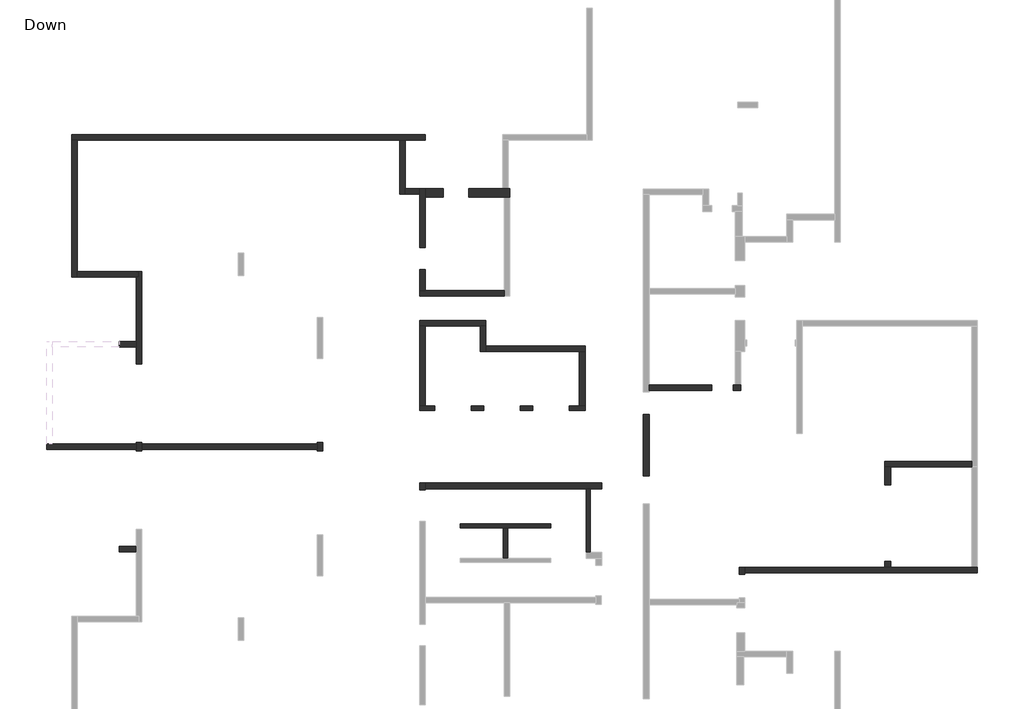
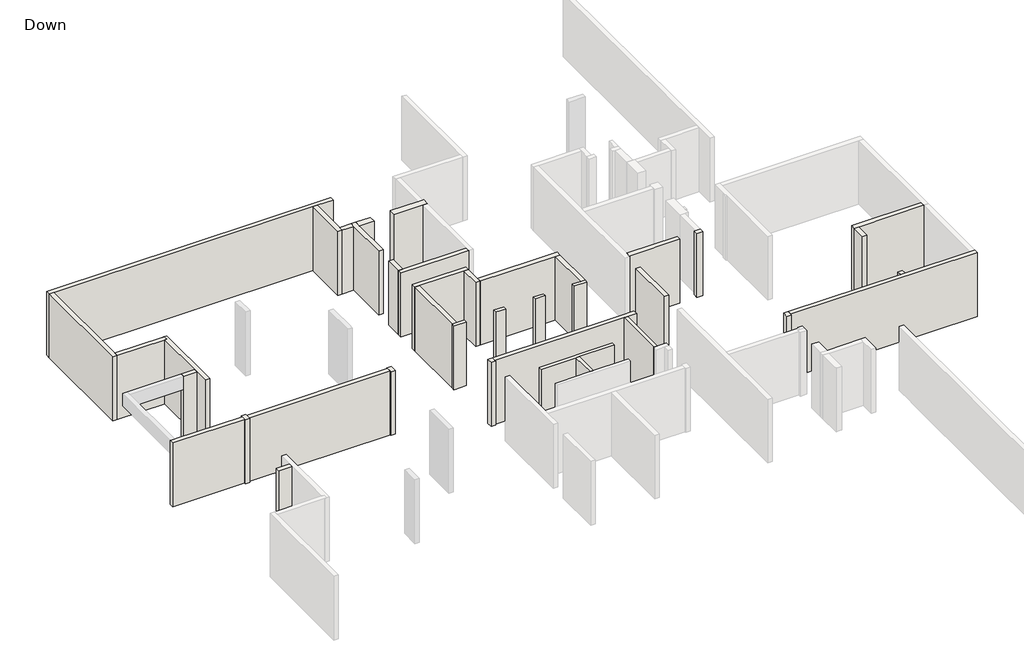
# One storey, part 2 of 3: 39 walls.
"""IFC4 building model written with IfcOpenShell, lengths in millimetres."""

from ifc_helpers import new_model, si_unit, origin, origin_with_axes, place, context, project, spatial, polyline, outline, extrude, faceted_brep, element, save

model = new_model("IFC4")

# Units and contexts
model_context = context("Model", 3, world=origin())
ifc_project = project(units=[si_unit("LENGTHUNIT", "METRE", prefix="MILLI")], contexts=[model_context])

# Site, building, storey
site = spatial("IfcSite", under=ifc_project)
building = spatial("IfcBuilding", under=site)
storey = spatial("IfcBuildingStorey", under=building, Name="Down", Elevation=0.0)

# Walls
placement = place(None, origin())
element("IfcWall", 1, ObjectType="15", at=placement, inside=storey, context=model_context, shape_type="Brep", body=[
    faceted_brep([(3274.3005639, 5124.0243454, 0.0), (3074.3005639, 5124.0243454, 0.0), (2715.3310352, 5124.0243454, 0.0), (2715.3310352, 5124.0243454, 2800.0), (2715.3310352, 5124.0243454, 3000.0), (3074.3005639, 5124.0243454, 3000.0), (3274.3005639, 5124.0243454, 3000.0), (3274.3005639, 4974.0243454, 0.0), (3274.3005639, 4974.0243454, 2800.0), (3274.3005639, 4974.0243454, 3000.0), (2715.3310352, 4974.0243454, 3000.0), (2715.3310352, 4974.0243454, 2800.0), (2715.3310352, 4974.0243454, 0.0)], [[[0, 1, 2, 3, 4, 5, 6]], [[7, 8, 9, 10, 11, 12]], [[2, 1, 0, 7, 12]], [[4, 3, 2, 12, 11, 10]], [[6, 5, 4, 10, 9]], [[0, 6, 9, 8, 7]]]),
])
element("IfcWall", 2, ObjectType="15", at=placement, inside=storey, context=model_context, shape_type="Brep", body=[
    faceted_brep([(1414.2577839, 5124.0243454, 0.0), (966.2691919, 5124.0243454, 0.0), (966.2691919, 5124.0243454, 2800.0), (966.2691919, 5124.0243454, 3000.0), (1414.2577839, 5124.0243454, 3000.0), (1414.2577839, 5124.0243454, 2800.0), (1414.2577839, 4974.0243454, 0.0), (1414.2577839, 4974.0243454, 2800.0), (1414.2577839, 4974.0243454, 3000.0), (966.2691919, 4974.0243454, 3000.0), (966.2691919, 4974.0243454, 2800.0), (966.2691919, 4974.0243454, 0.0)], [[[0, 1, 2, 3, 4, 5]], [[6, 7, 8, 9, 10, 11]], [[1, 0, 6, 11]], [[3, 2, 1, 11, 10, 9]], [[4, 3, 9, 8]], [[0, 5, 4, 8, 7, 6]]]),
])
element("IfcWall", 3, ObjectType="15", at=placement, inside=storey, context=model_context, shape_type="Brep", body=[
    faceted_brep([(-334.8040593, 5124.0243454, 0.0), (-785.1755694, 5124.0243454, 0.0), (-785.1755694, 5124.0243454, 2800.0), (-785.1755694, 5124.0243454, 3000.0), (-334.8040593, 5124.0243454, 3000.0), (-334.8040593, 5124.0243454, 2800.0), (-334.8040593, 4974.0243454, 0.0), (-334.8040593, 4974.0243454, 2800.0), (-334.8040593, 4974.0243454, 3000.0), (-785.1755694, 4974.0243454, 3000.0), (-785.1755694, 4974.0243454, 2800.0), (-785.1755694, 4974.0243454, 0.0)], [[[0, 1, 2, 3, 4, 5]], [[6, 7, 8, 9, 10, 11]], [[1, 0, 6, 11]], [[3, 2, 1, 11, 10, 9]], [[4, 3, 9, 8]], [[0, 5, 4, 8, 7, 6]]]),
])
element("IfcWall", 4, ObjectType="15", at=placement, inside=storey, context=model_context, shape_type="Brep", body=[
    faceted_brep([(-2083.8659026, 5124.0243454, 0.0), (-2434.3199705, 5124.0243454, 0.0), (-2634.3199705, 5124.0243454, 0.0), (-2634.3199705, 5124.0243454, 3000.0), (-2434.3199705, 5124.0243454, 3000.0), (-2083.8659026, 5124.0243454, 3000.0), (-2083.8659026, 5124.0243454, 2800.0), (-2083.8659026, 4974.0243454, 0.0), (-2083.8659026, 4974.0243454, 2800.0), (-2083.8659026, 4974.0243454, 3000.0), (-2634.3199705, 4974.0243454, 3000.0), (-2634.3199705, 4974.0243454, 2800.0), (-2634.3199705, 4974.0243454, 0.0)], [[[0, 1, 2, 3, 4, 5, 6]], [[7, 8, 9, 10, 11, 12]], [[2, 1, 0, 7, 12]], [[5, 4, 3, 10, 9]], [[0, 6, 5, 9, 8, 7]], [[3, 2, 12, 11, 10]]]),
])
element("IfcWall", 5, ObjectType="15", at=placement, inside=storey, context=model_context, shape_type="Brep", body=[
    faceted_brep([(3311.0605459, 2174.0956453, 0.0), (3311.0605459, -105.9043547, 0.0), (3311.0605459, -105.9043547, 3000.0), (3311.0605459, 2174.0956453, 3000.0), (3461.0605459, 2174.0956453, 0.0), (3461.0605459, 2174.0956453, 3000.0), (3461.0605459, -105.9043547, 3000.0), (3461.0605459, -105.9043547, 2800.0), (3461.0605459, -105.9043547, 0.0)], [[[0, 1, 2, 3]], [[4, 5, 6, 7, 8]], [[1, 0, 4, 8]], [[3, 2, 6, 5]], [[0, 3, 5, 4]], [[2, 1, 8, 7, 6]]]),
])
element("IfcWall", 6, ObjectType="15", at=placement, inside=storey, context=model_context, shape_type="Brep", body=[
    faceted_brep([(-1185.5058006, 773.063673, 0.0), (361.0080091, 773.063673, 0.0), (511.0080091, 773.063673, 0.0), (2055.2627374, 773.063673, 0.0), (2055.2627374, 773.063673, 2800.0), (2055.2627374, 773.063673, 3000.0), (1795.2627374, 773.063673, 3000.0), (511.0080091, 773.063673, 3000.0), (361.0080091, 773.063673, 3000.0), (-985.5058006, 773.063673, 3000.0), (-1185.5058006, 773.063673, 3000.0), (-1185.5058006, 773.063673, 2800.0), (-1185.5058006, 923.063673, 0.0), (-1185.5058006, 923.063673, 2800.0), (-1185.5058006, 923.063673, 3000.0), (2055.2627374, 923.063673, 3000.0), (2055.2627374, 923.063673, 2800.0), (2055.2627374, 923.063673, 0.0)], [[[0, 1, 2, 3, 4, 5, 6, 7, 8, 9, 10, 11]], [[12, 13, 14, 15, 16, 17]], [[3, 2, 1, 0, 12, 17]], [[5, 4, 3, 17, 16, 15]], [[10, 9, 8, 7, 6, 5, 15, 14]], [[0, 11, 10, 14, 13, 12]]]),
])
element("IfcWall", 7, ObjectType="15", at=placement, inside=storey, context=model_context, shape_type="SweptSolid", body=[
    extrude(outline(polyline([(511.0080091, 773.063673), (511.0080091, -306.6458737), (361.0080091, -306.6458737), (361.0080091, 773.063673), (511.0080091, 773.063673)])), origin_with_axes(), (0.0, 0.0, 1.0), 3000.0),
])
element("IfcWall", 8, ObjectType="20", at=placement, inside=storey, context=model_context, shape_type="Brep", body=[
    faceted_brep([(5555.6042265, 5674.60225, 0.0), (7795.7123021, 5674.60225, 0.0), (7795.7123021, 5674.60225, 2800.0), (7795.7123021, 5674.60225, 3000.0), (5555.6042265, 5674.60225, 3000.0), (5555.6042265, 5674.60225, 2800.0), (5555.6042265, 5874.60225, 0.0), (5555.6042265, 5874.60225, 2800.0), (5555.6042265, 5874.60225, 3000.0), (7795.7123021, 5874.60225, 3000.0), (7795.7123021, 5874.60225, 2800.0), (7795.7123021, 5874.60225, 0.0)], [[[0, 1, 2, 3, 4, 5]], [[6, 7, 8, 9, 10, 11]], [[1, 0, 6, 11]], [[3, 2, 1, 11, 10, 9]], [[4, 3, 9, 8]], [[0, 5, 4, 8, 7, 6]]]),
])
element("IfcWall", 9, ObjectType="20", at=placement, inside=storey, context=model_context, shape_type="Brep", body=[
    faceted_brep([(8565.3948299, 5674.60225, 0.0), (8829.8987326, 5674.60225, 0.0), (8829.8987326, 5674.60225, 2800.0), (8829.8987326, 5674.60225, 3000.0), (8565.3948299, 5674.60225, 3000.0), (8565.3948299, 5674.60225, 2800.0), (8565.3948299, 5874.60225, 0.0), (8565.3948299, 5874.60225, 2800.0), (8565.3948299, 5874.60225, 3000.0), (8629.8987326, 5874.60225, 3000.0), (8829.8987326, 5874.60225, 3000.0), (8829.8987326, 5874.60225, 0.0), (8629.8987326, 5874.60225, 0.0)], [[[0, 1, 2, 3, 4, 5]], [[6, 7, 8, 9, 10, 11, 12]], [[1, 0, 6, 12, 11]], [[4, 3, 10, 9, 8]], [[0, 5, 4, 8, 7, 6]], [[3, 2, 1, 11, 10]]]),
])
element("IfcWall", 10, ObjectType="20", at=placement, inside=storey, context=model_context, shape_type="Brep", body=[
    faceted_brep([(17074.9602757, 3143.7781731, 0.0), (13974.6187866, 3143.7781731, 0.0), (13974.6187866, 3143.7781731, 2800.0), (13974.6187866, 3143.7781731, 3000.0), (17074.9602757, 3143.7781731, 3000.0), (17074.9602757, 3143.7781731, 2800.0), (17074.9602757, 2943.7781731, 0.0), (17074.9602757, 2943.7781731, 2800.0), (17074.9602757, 2943.7781731, 3000.0), (14174.6187866, 2943.7781731, 3000.0), (13974.6187866, 2943.7781731, 3000.0), (13974.6187866, 2943.7781731, 0.0), (14174.6187866, 2943.7781731, 0.0)], [[[0, 1, 2, 3, 4, 5]], [[6, 7, 8, 9, 10, 11, 12]], [[1, 0, 6, 12, 11]], [[4, 3, 10, 9, 8]], [[0, 5, 4, 8, 7, 6]], [[3, 2, 1, 11, 10]]]),
])
element("IfcWall", 11, ObjectType="20", at=placement, inside=storey, context=model_context, shape_type="Brep", body=[
    faceted_brep([(13974.6187866, 2943.7781731, 0.0), (13974.6187866, 2314.6878099, 0.0), (13974.6187866, 2314.6878099, 2800.0), (13974.6187866, 2314.6878099, 3000.0), (13974.6187866, 2943.7781731, 3000.0), (14174.6187866, 2943.7781731, 0.0), (14174.6187866, 2943.7781731, 2800.0), (14174.6187866, 2943.7781731, 3000.0), (14174.6187866, 2314.6878099, 3000.0), (14174.6187866, 2314.6878099, 2800.0), (14174.6187866, 2314.6878099, 0.0)], [[[0, 1, 2, 3, 4]], [[5, 6, 7, 8, 9, 10]], [[1, 0, 5, 10]], [[3, 2, 1, 10, 9, 8]], [[4, 3, 8, 7]], [[0, 4, 7, 6, 5]]]),
])
element("IfcWall", 12, ObjectType="20", at=placement, inside=storey, context=model_context, shape_type="Brep", body=[
    faceted_brep([(-2431.7719369, 14822.6246156, 0.0), (-15051.7058906, 14822.6246156, 0.0), (-15051.7058906, 14822.6246156, 3000.0), (-2431.7719369, 14822.6246156, 3000.0), (-2431.7719369, 14622.6246156, 0.0), (-2431.7719369, 14622.6246156, 3000.0), (-3134.897875, 14622.6246156, 3000.0), (-3334.897875, 14622.6246156, 3000.0), (-14851.7058906, 14622.6246156, 3000.0), (-15051.7058906, 14622.6246156, 3000.0), (-15051.7058906, 14622.6246156, 0.0), (-14851.7058906, 14622.6246156, 0.0), (-3334.897875, 14622.6246156, 0.0), (-3134.897875, 14622.6246156, 0.0)], [[[0, 1, 2, 3]], [[4, 5, 6, 7, 8, 9, 10, 11, 12, 13]], [[1, 0, 4, 13, 12, 11, 10]], [[3, 2, 9, 8, 7, 6, 5]], [[0, 3, 5, 4]], [[2, 1, 10, 9]]]),
])
element("IfcWall", 13, ObjectType="20", at=placement, inside=storey, context=model_context, shape_type="Brep", body=[
    faceted_brep([(-15051.7058906, 14622.6246156, 0.0), (-15051.7058906, 9722.6246156, 0.0), (-15051.7058906, 9722.6246156, 3000.0), (-15051.7058906, 14622.6246156, 3000.0), (-14851.7058906, 14622.6246156, 0.0), (-14851.7058906, 14622.6246156, 2800.0), (-14851.7058906, 14622.6246156, 3000.0), (-14851.7058906, 9922.6246156, 3000.0), (-14851.7058906, 9722.6246156, 3000.0), (-14851.7058906, 9722.6246156, 0.0), (-14851.7058906, 9922.6246156, 0.0)], [[[0, 1, 2, 3]], [[4, 5, 6, 7, 8, 9, 10]], [[1, 0, 4, 10, 9]], [[3, 2, 8, 7, 6]], [[0, 3, 6, 5, 4]], [[2, 1, 9, 8]]]),
])
element("IfcWall", 14, ObjectType="20", at=placement, inside=storey, context=model_context, shape_type="Brep", body=[
    faceted_brep([(-14851.7058906, 9722.6246156, 0.0), (-12744.8761098, 9722.6246156, 0.0), (-12645.0412254, 9722.6246156, 0.0), (-12645.0412254, 9722.6246156, 3000.0), (-12744.8761098, 9722.6246156, 3000.0), (-14851.7058906, 9722.6246156, 3000.0), (-14851.7058906, 9922.6246156, 0.0), (-14851.7058906, 9922.6246156, 2800.0), (-14851.7058906, 9922.6246156, 3000.0), (-12744.8761098, 9922.6246156, 3000.0), (-12645.0412254, 9922.6246156, 3000.0), (-12645.0412254, 9922.6246156, 0.0), (-12744.8761098, 9922.6246156, 0.0)], [[[0, 1, 2, 3, 4, 5]], [[6, 7, 8, 9, 10, 11, 12]], [[2, 1, 0, 6, 12, 11]], [[3, 2, 11, 10]], [[5, 4, 3, 10, 9, 8]], [[0, 5, 8, 7, 6]]]),
])
element("IfcWall", 15, ObjectType="20", at=placement, inside=storey, context=model_context, shape_type="Brep", body=[
    faceted_brep([(-12744.8761098, 6623.0036309, 0.0), (-12744.8761098, 6623.0036309, 2800.0), (-12744.8761098, 6623.0036309, 3000.0), (-12744.8761098, 7228.4299293, 3000.0), (-12744.8761098, 7428.4299293, 3000.0), (-12744.8761098, 9722.6246156, 3000.0), (-12744.8761098, 9722.6246156, 0.0), (-12744.8761098, 7428.4299293, 0.0), (-12744.8761098, 7228.4299293, 0.0), (-12744.8761098, 9923.0036309, 3000.0), (-12744.8761098, 9923.0036309, 2800.0), (-12744.8761098, 9923.0036309, 0.0), (-12744.8761098, 9922.6246156, 0.0), (-12744.8761098, 9922.6246156, 2800.0), (-12744.8761098, 9922.6246156, 3000.0), (-12544.8761098, 6623.0036309, 0.0), (-12544.8761098, 9923.0036309, 0.0), (-12544.8761098, 9923.0036309, 2800.0), (-12544.8761098, 9923.0036309, 3000.0), (-12544.8761098, 6623.0036309, 3000.0), (-12544.8761098, 6623.0036309, 2800.0), (-12645.0412254, 9722.6246156, 0.0), (-12645.0412254, 9922.6246156, 0.0), (-12742.9172386, 6623.0036309, 3000.0), (-12645.0412254, 9922.6246156, 3000.0), (-12645.0412254, 9722.6246156, 3000.0)], [[[0, 1, 2, 3, 4, 5, 6, 7, 8]], [[9, 10, 11, 12, 13, 14]], [[15, 16, 17, 18, 19, 20]], [[16, 15, 0, 8, 7, 6, 21, 22, 12, 11]], [[2, 1, 0, 15, 20, 19, 23]], [[19, 18, 9, 14, 24, 25, 5, 4, 3, 2, 23]], [[11, 10, 9, 18, 17, 16]], [[25, 21, 6, 5]], [[22, 24, 14, 13, 12]], [[21, 25, 24, 22]]]),
])
element("IfcWall", 16, ObjectType="20", at=placement, inside=storey, context=model_context, shape_type="Brep", body=[
    faceted_brep([(-12744.8761098, 7428.4299293, 0.0), (-13340.0412254, 7428.4299293, 0.0), (-13340.0412254, 7428.4299293, 2400.0), (-13340.0412254, 7428.4299293, 3000.0), (-12744.8761098, 7428.4299293, 3000.0), (-12744.8761098, 7228.4299293, 0.0), (-12744.8761098, 7228.4299293, 2800.0), (-12744.8761098, 7228.4299293, 3000.0), (-13340.0412254, 7228.4299293, 3000.0), (-13340.0412254, 7228.4299293, 2400.0), (-13340.0412254, 7228.4299293, 0.0)], [[[0, 1, 2, 3, 4]], [[5, 6, 7, 8, 9, 10]], [[1, 0, 5, 10]], [[3, 2, 1, 10, 9, 8]], [[4, 3, 8, 7]], [[0, 4, 7, 6, 5]]]),
])
element("IfcWall", 17, ObjectType="20", at=placement, inside=storey, context=model_context, shape_type="Brep", body=[
    faceted_brep([(-15942.9172386, 3570.6507339, 0.0), (-12745.0412254, 3570.6507339, 0.0), (-12742.9172386, 3570.6507339, 0.0), (-12742.9172386, 3570.6507339, 3000.0), (-12745.0412254, 3570.6507339, 3000.0), (-15742.9172386, 3570.6507339, 3000.0), (-15942.9172386, 3570.6507339, 3000.0), (-15942.9172386, 3770.6507339, 0.0), (-15942.9172386, 3770.6507339, 3000.0), (-15742.9172386, 3770.6507339, 3000.0), (-12745.0412254, 3770.6507339, 3000.0), (-12742.9172386, 3770.6507339, 3000.0), (-12742.9172386, 3770.6507339, 0.0), (-12745.0412254, 3770.6507339, 0.0)], [[[0, 1, 2, 3, 4, 5, 6]], [[7, 8, 9, 10, 11, 12, 13]], [[2, 1, 0, 7, 13, 12]], [[3, 2, 12, 11]], [[6, 5, 4, 3, 11, 10, 9, 8]], [[0, 6, 8, 7]]]),
])
element("IfcWall", 18, ObjectType="20", at=placement, inside=storey, context=model_context, shape_type="Brep", body=[
    faceted_brep([(-12745.0412254, 3522.8272575, 0.0), (-12745.0412254, 3522.8272575, 2800.0), (-12745.0412254, 3522.8272575, 3000.0), (-12745.0412254, 3570.6507339, 3000.0), (-12745.0412254, 3570.6507339, 2800.0), (-12745.0412254, 3570.6507339, 0.0), (-12745.0412254, 3818.3090948, 3000.0), (-12745.0412254, 3818.3090948, 2800.0), (-12745.0412254, 3818.3090948, 0.0), (-12745.0412254, 3770.6507339, 0.0), (-12745.0412254, 3770.6507339, 2800.0), (-12745.0412254, 3770.6507339, 3000.0), (-12545.0412254, 3522.8272575, 0.0), (-12545.0412254, 3573.033652, 0.0), (-12545.0412254, 3773.033652, 0.0), (-12545.0412254, 3818.3090948, 0.0), (-12545.0412254, 3818.3090948, 3000.0), (-12545.0412254, 3773.033652, 3000.0), (-12545.0412254, 3573.033652, 3000.0), (-12545.0412254, 3522.8272575, 3000.0), (-12545.0412254, 3522.8272575, 2800.0), (-12742.9172386, 3570.6507339, 0.0), (-12742.9172386, 3770.6507339, 0.0), (-12744.8761098, 3522.8272575, 3000.0), (-12742.9172386, 3818.3090948, 3000.0), (-12742.9172386, 3770.6507339, 3000.0), (-12742.9172386, 3570.6507339, 3000.0)], [[[0, 1, 2, 3, 4, 5]], [[6, 7, 8, 9, 10, 11]], [[12, 13, 14, 15, 16, 17, 18, 19, 20]], [[15, 14, 13, 12, 0, 5, 21, 22, 9, 8]], [[2, 1, 0, 12, 20, 19, 23]], [[19, 18, 17, 16, 24, 6, 11, 25, 26, 3, 2, 23]], [[8, 7, 6, 24, 16, 15]], [[26, 21, 5, 4, 3]], [[22, 25, 11, 10, 9]], [[21, 26, 25, 22]]]),
])
element("IfcWall", 19, ObjectType="20", at=placement, inside=storey, context=model_context, shape_type="Brep", body=[
    faceted_brep([(-12545.0412254, 3573.033652, 0.0), (-6284.9504118, 3573.033652, 0.0), (-6284.9504118, 3573.033652, 2800.0), (-6284.9504118, 3573.033652, 3000.0), (-12545.0412254, 3573.033652, 3000.0), (-12545.0412254, 3573.033652, 2800.0), (-12545.0412254, 3773.033652, 0.0), (-12545.0412254, 3773.033652, 2800.0), (-12545.0412254, 3773.033652, 3000.0), (-6284.9504118, 3773.033652, 3000.0), (-6284.9504118, 3773.033652, 2800.0), (-6284.9504118, 3773.033652, 0.0)], [[[0, 1, 2, 3, 4, 5]], [[6, 7, 8, 9, 10, 11]], [[1, 0, 6, 11]], [[4, 3, 9, 8]], [[0, 5, 4, 8, 7, 6]], [[3, 2, 1, 11, 10, 9]]]),
])
element("IfcWall", 20, ObjectType="20", at=placement, inside=storey, context=model_context, shape_type="Brep", body=[
    faceted_brep([(-6284.9504118, 3823.0749308, 0.0), (-6284.9504118, 3773.033652, 0.0), (-6284.9504118, 3573.033652, 0.0), (-6284.9504118, 3522.8272575, 0.0), (-6284.9504118, 3522.8272575, 2800.0), (-6284.9504118, 3522.8272575, 3000.0), (-6284.9504118, 3573.033652, 3000.0), (-6284.9504118, 3773.033652, 3000.0), (-6284.9504118, 3823.0749308, 3000.0), (-6084.9504118, 3823.0749308, 0.0), (-6084.9504118, 3823.0749308, 3000.0), (-6084.9504118, 3672.9510942, 3000.0), (-6084.9504118, 3522.8272575, 3000.0), (-6084.9504118, 3522.8272575, 2800.0), (-6084.9504118, 3522.8272575, 0.0)], [[[0, 1, 2, 3, 4, 5, 6, 7, 8]], [[9, 10, 11, 12, 13, 14]], [[3, 2, 1, 0, 9, 14]], [[5, 4, 3, 14, 13, 12]], [[8, 7, 6, 5, 12, 11, 10]], [[0, 8, 10, 9]]]),
])
element("IfcWall", 21, ObjectType="20", at=placement, inside=storey, context=model_context, shape_type="Brep", body=[
    faceted_brep([(-3134.897875, 12692.2958855, 0.0), (-3134.897875, 12892.2958855, 0.0), (-3134.897875, 14622.6246156, 0.0), (-3134.897875, 14622.6246156, 3000.0), (-3134.897875, 12892.2958855, 3000.0), (-3134.897875, 12692.2958855, 3000.0), (-3334.897875, 12692.2958855, 0.0), (-3334.897875, 12692.2958855, 2800.0), (-3334.897875, 12692.2958855, 3000.0), (-3334.897875, 14622.6246156, 3000.0), (-3334.897875, 14622.6246156, 2800.0), (-3334.897875, 14622.6246156, 0.0)], [[[0, 1, 2, 3, 4, 5]], [[6, 7, 8, 9, 10, 11]], [[2, 1, 0, 6, 11]], [[5, 4, 3, 9, 8]], [[0, 5, 8, 7, 6]], [[3, 2, 11, 10, 9]]]),
])
element("IfcWall", 22, ObjectType="20", at=placement, inside=storey, context=model_context, shape_type="Brep", body=[
    faceted_brep([(-3134.897875, 12692.2958855, 0.0), (-2634.3199705, 12692.2958855, 0.0), (-2634.3199705, 12692.2958855, 2800.0), (-2634.3199705, 12692.2958855, 3000.0), (-3134.897875, 12692.2958855, 3000.0), (-3134.897875, 12892.2958855, 0.0), (-3134.897875, 12892.2958855, 3000.0), (-2634.3199705, 12892.2958855, 3000.0), (-2634.3199705, 12892.2958855, 0.0)], [[[0, 1, 2, 3, 4]], [[5, 6, 7, 8]], [[1, 0, 5, 8]], [[4, 3, 7, 6]], [[0, 4, 6, 5]], [[3, 2, 1, 8, 7]]]),
])
element("IfcWall", 23, ObjectType="20", at=placement, inside=storey, context=model_context, shape_type="Brep", body=[
    faceted_brep([(-2434.3199705, 10776.4297792, 0.0), (-2434.3199705, 12592.2958855, 0.0), (-2434.3199705, 12892.2958855, 0.0), (-2434.3199705, 12892.2958855, 3000.0), (-2434.3199705, 12592.2958855, 3000.0), (-2434.3199705, 10776.4297792, 3000.0), (-2434.3199705, 10776.4297792, 2800.0), (-2634.3199705, 10776.4297792, 0.0), (-2634.3199705, 10776.4297792, 2800.0), (-2634.3199705, 10776.4297792, 3000.0), (-2634.3199705, 12692.2958855, 3000.0), (-2634.3199705, 12892.2958855, 3000.0), (-2634.3199705, 12892.2958855, 0.0), (-2634.3199705, 12692.2958855, 0.0)], [[[0, 1, 2, 3, 4, 5, 6]], [[7, 8, 9, 10, 11, 12, 13]], [[2, 1, 0, 7, 13, 12]], [[5, 4, 3, 11, 10, 9]], [[0, 6, 5, 9, 8, 7]], [[3, 2, 12, 11]]]),
])
element("IfcWall", 24, ObjectType="20", at=placement, inside=storey, context=model_context, shape_type="Brep", body=[
    faceted_brep([(385.0023051, 9253.5800344, 0.0), (-2434.3199705, 9253.5800344, 0.0), (-2634.3199705, 9253.5800344, 0.0), (-2634.3199705, 9253.5800344, 3000.0), (-2434.3199705, 9253.5800344, 3000.0), (385.0023051, 9253.5800344, 3000.0), (385.0023051, 9253.5800344, 2800.0), (385.0023051, 9053.5800344, 0.0), (385.0023051, 9053.5800344, 3000.0), (-463.4816337, 9053.5800344, 3000.0), (-2634.3199705, 9053.5800344, 3000.0), (-2634.3199705, 9053.5800344, 0.0)], [[[0, 1, 2, 3, 4, 5, 6]], [[7, 8, 9, 10, 11]], [[2, 1, 0, 7, 11]], [[5, 4, 3, 10, 9, 8]], [[0, 6, 5, 8, 7]], [[3, 2, 11, 10]]]),
])
element("IfcWall", 25, ObjectType="20", at=placement, inside=storey, context=model_context, shape_type="Brep", body=[
    faceted_brep([(-2434.3199705, 9253.5800344, 0.0), (-2434.3199705, 10006.7472515, 0.0), (-2434.3199705, 10006.7472515, 2800.0), (-2434.3199705, 10006.7472515, 3000.0), (-2434.3199705, 9253.5800344, 3000.0), (-2434.3199705, 9253.5800344, 2800.0), (-2634.3199705, 9253.5800344, 0.0), (-2634.3199705, 9253.5800344, 3000.0), (-2634.3199705, 10006.7472515, 3000.0), (-2634.3199705, 10006.7472515, 2800.0), (-2634.3199705, 10006.7472515, 0.0)], [[[0, 1, 2, 3, 4, 5]], [[6, 7, 8, 9, 10]], [[1, 0, 6, 10]], [[3, 2, 1, 10, 9, 8]], [[4, 3, 8, 7]], [[0, 5, 4, 7, 6]]]),
])
element("IfcWall", 26, ObjectType="20", at=placement, inside=storey, context=model_context, shape_type="Brep", body=[
    faceted_brep([(8979.8574537, -828.2159728, 0.0), (17274.9602757, -828.2159728, 0.0), (17274.9602757, -828.2159728, 3000.0), (8979.8574537, -828.2159728, 3000.0), (8979.8574537, -628.2159728, 0.0), (8979.8574537, -628.2159728, 3000.0), (13974.6187866, -628.2159728, 3000.0), (14174.6187866, -628.2159728, 3000.0), (17074.9602757, -628.2159728, 3000.0), (17274.9602757, -628.2159728, 3000.0), (17274.9602757, -628.2159728, 0.0), (17074.9602757, -628.2159728, 0.0), (14174.6187866, -628.2159728, 0.0), (13974.6187866, -628.2159728, 0.0)], [[[0, 1, 2, 3]], [[4, 5, 6, 7, 8, 9, 10, 11, 12, 13]], [[1, 0, 4, 13, 12, 11, 10]], [[3, 2, 9, 8, 7, 6, 5]], [[2, 1, 10, 9]], [[0, 3, 5, 4]]]),
])
element("IfcWall", 27, ObjectType="20", at=placement, inside=storey, context=model_context, shape_type="Brep", body=[
    faceted_brep([(-12744.8761098, 117.6373746, 0.0), (-13340.0412254, 117.6373746, 0.0), (-13340.0412254, 117.6373746, 2400.0), (-13340.0412254, 117.6373746, 3000.0), (-12744.8761098, 117.6373746, 3000.0), (-12744.8761098, 117.6373746, 2800.0), (-12744.8761098, -82.3626254, 0.0), (-12744.8761098, -82.3626254, 3000.0), (-13340.0412254, -82.3626254, 3000.0), (-13340.0412254, -82.3626254, 2400.0), (-13340.0412254, -82.3626254, 0.0)], [[[0, 1, 2, 3, 4, 5]], [[6, 7, 8, 9, 10]], [[1, 0, 6, 10]], [[3, 2, 1, 10, 9, 8]], [[4, 3, 8, 7]], [[0, 5, 4, 7, 6]]]),
])
element("IfcWall", 28, ObjectType="20", at=placement, inside=storey, context=model_context, shape_type="Brep", body=[
    faceted_brep([(5355.6042265, 4823.9005088, 0.0), (5355.6042265, 2624.4671554, 0.0), (5355.6042265, 2624.4671554, 2800.0), (5355.6042265, 2624.4671554, 3000.0), (5355.6042265, 4823.9005088, 3000.0), (5355.6042265, 4823.9005088, 2800.0), (5555.6042265, 4823.9005088, 0.0), (5555.6042265, 4823.9005088, 2800.0), (5555.6042265, 4823.9005088, 3000.0), (5555.6042265, 2624.4671554, 3000.0), (5555.6042265, 2624.4671554, 2800.0), (5555.6042265, 2624.4671554, 0.0)], [[[0, 1, 2, 3, 4, 5]], [[6, 7, 8, 9, 10, 11]], [[1, 0, 6, 11]], [[3, 2, 1, 11, 10, 9]], [[4, 3, 9, 8]], [[0, 5, 4, 8, 7, 6]]]),
])
element("IfcWall", 29, ObjectType="20", at=placement, inside=storey, context=model_context, shape_type="Brep", body=[
    faceted_brep([(8779.8574537, -628.2159728, 0.0), (8779.8574537, -878.4223673, 0.0), (8779.8574537, -878.4223673, 2800.0), (8779.8574537, -878.4223673, 3000.0), (8779.8574537, -628.2159728, 3000.0), (8779.8574537, -628.2159728, 2800.0), (8979.8574537, -628.2159728, 0.0), (8979.8574537, -628.2159728, 3000.0), (8979.8574537, -828.2159728, 3000.0), (8979.8574537, -878.4223673, 3000.0), (8979.8574537, -878.4223673, 2800.0), (8979.8574537, -878.4223673, 0.0), (8979.8574537, -828.2159728, 0.0)], [[[0, 1, 2, 3, 4, 5]], [[6, 7, 8, 9, 10, 11, 12]], [[1, 0, 6, 12, 11]], [[3, 2, 1, 11, 10, 9]], [[4, 3, 9, 8, 7]], [[0, 5, 4, 7, 6]]]),
])
element("IfcWall", 30, ObjectType="20", at=placement, inside=storey, context=model_context, shape_type="Brep", body=[
    faceted_brep([(13974.6187866, -425.6679392, 0.0), (13974.6187866, -628.2159728, 0.0), (13974.6187866, -628.2159728, 2800.0), (13974.6187866, -628.2159728, 3000.0), (13974.6187866, -425.6679392, 3000.0), (13974.6187866, -425.6679392, 2800.0), (14174.6187866, -425.6679392, 0.0), (14174.6187866, -425.6679392, 2800.0), (14174.6187866, -425.6679392, 3000.0), (14174.6187866, -628.2159728, 3000.0), (14174.6187866, -628.2159728, 2800.0), (14174.6187866, -628.2159728, 0.0)], [[[0, 1, 2, 3, 4, 5]], [[6, 7, 8, 9, 10, 11]], [[1, 0, 6, 11]], [[4, 3, 9, 8]], [[0, 5, 4, 8, 7, 6]], [[3, 2, 1, 11, 10, 9]]]),
])
element("IfcWall", 31, ObjectType="20", at=placement, inside=storey, context=model_context, shape_type="Brep", body=[
    faceted_brep([(-2634.3199705, 7974.2832767, 0.0), (-2434.3199705, 7974.2832767, 0.0), (-465.6994361, 7974.2832767, 0.0), (-265.6994361, 7974.2832767, 0.0), (-265.6994361, 7974.2832767, 3000.0), (-465.6994361, 7974.2832767, 3000.0), (-2434.3199705, 7974.2832767, 3000.0), (-2634.3199705, 7974.2832767, 3000.0), (-2634.3199705, 8174.2832767, 0.0), (-2634.3199705, 8174.2832767, 3000.0), (-463.4816337, 8174.2832767, 3000.0), (-265.6994361, 8174.2832767, 3000.0), (-265.6994361, 8174.2832767, 2800.0), (-265.6994361, 8174.2832767, 0.0)], [[[0, 1, 2, 3, 4, 5, 6, 7]], [[8, 9, 10, 11, 12, 13]], [[3, 2, 1, 0, 8, 13]], [[7, 6, 5, 4, 11, 10, 9]], [[4, 3, 13, 12, 11]], [[0, 7, 9, 8]]]),
])
element("IfcWall", 32, ObjectType="20", at=placement, inside=storey, context=model_context, shape_type="Brep", body=[
    faceted_brep([(-465.6994361, 7974.2832767, 0.0), (-465.6994361, 7073.375141, 0.0), (-465.6994361, 7073.375141, 3000.0), (-465.6994361, 7974.2832767, 3000.0), (-265.6994361, 7974.2832767, 0.0), (-265.6994361, 7974.2832767, 3000.0), (-265.6994361, 7273.375141, 3000.0), (-265.6994361, 7073.375141, 3000.0), (-265.6994361, 7073.375141, 0.0), (-265.6994361, 7273.375141, 0.0)], [[[0, 1, 2, 3]], [[4, 5, 6, 7, 8, 9]], [[1, 0, 4, 9, 8]], [[3, 2, 7, 6, 5]], [[0, 3, 5, 4]], [[2, 1, 8, 7]]]),
])
element("IfcWall", 33, ObjectType="20", at=placement, inside=storey, context=model_context, shape_type="Brep", body=[
    faceted_brep([(-265.6994361, 7073.375141, 0.0), (3074.3005639, 7073.375141, 0.0), (3274.3005639, 7073.375141, 0.0), (3274.3005639, 7073.375141, 3000.0), (3074.3005639, 7073.375141, 3000.0), (-265.6994361, 7073.375141, 3000.0), (-265.6994361, 7273.375141, 0.0), (-265.6994361, 7273.375141, 2800.0), (-265.6994361, 7273.375141, 3000.0), (3274.3005639, 7273.375141, 3000.0), (3274.3005639, 7273.375141, 2800.0), (3274.3005639, 7273.375141, 0.0)], [[[0, 1, 2, 3, 4, 5]], [[6, 7, 8, 9, 10, 11]], [[2, 1, 0, 6, 11]], [[5, 4, 3, 9, 8]], [[0, 5, 8, 7, 6]], [[3, 2, 11, 10, 9]]]),
])
element("IfcWall", 34, ObjectType="20", at=placement, inside=storey, context=model_context, shape_type="SweptSolid", body=[
    extrude(outline(polyline([(3074.3005639, 5124.0243454), (3074.3005639, 7073.375141), (3274.3005639, 7073.375141), (3274.3005639, 5124.0243454), (3074.3005639, 5124.0243454)])), origin_with_axes(), (0.0, 0.0, 1.0), 3000.0),
])
element("IfcWall", 35, ObjectType="20", at=placement, inside=storey, context=model_context, shape_type="SweptSolid", body=[
    extrude(outline(polyline([(-2434.3199705, 7974.2832767), (-2434.3199705, 5124.0243454), (-2634.3199705, 5124.0243454), (-2634.3199705, 7974.2832767), (-2434.3199705, 7974.2832767)])), origin_with_axes(), (0.0, 0.0, 1.0), 3000.0),
])
element("IfcWall", 36, ObjectType="20", at=placement, inside=storey, context=model_context, shape_type="Brep", body=[
    faceted_brep([(-2434.3199705, 2124.0543665, 0.0), (-2434.3199705, 2174.2607609, 0.0), (-2434.3199705, 2374.2607609, 0.0), (-2434.3199705, 2374.2607609, 3000.0), (-2434.3199705, 2174.2607609, 3000.0), (-2434.3199705, 2124.0543665, 3000.0), (-2434.3199705, 2124.0543665, 2800.0), (-2634.3199705, 2124.0543665, 0.0), (-2634.3199705, 2124.0543665, 2800.0), (-2634.3199705, 2124.0543665, 3000.0), (-2634.3199705, 2374.2607609, 3000.0), (-2634.3199705, 2374.2607609, 2800.0), (-2634.3199705, 2374.2607609, 0.0)], [[[0, 1, 2, 3, 4, 5, 6]], [[7, 8, 9, 10, 11, 12]], [[2, 1, 0, 7, 12]], [[5, 4, 3, 10, 9]], [[0, 6, 5, 9, 8, 7]], [[3, 2, 12, 11, 10]]]),
])
element("IfcWall", 37, ObjectType="20", at=placement, inside=storey, context=model_context, shape_type="Brep", body=[
    faceted_brep([(-2434.3199705, 2174.2607609, 0.0), (3861.5146137, 2174.2607609, 0.0), (3861.5146137, 2174.2607609, 2800.0), (3861.5146137, 2174.2607609, 3000.0), (3461.0605459, 2174.2607609, 3000.0), (3311.0605459, 2174.2607609, 3000.0), (-2434.3199705, 2174.2607609, 3000.0), (-2434.3199705, 2174.2607609, 2800.0), (-2434.3199705, 2374.2607609, 0.0), (-2434.3199705, 2374.2607609, 3000.0), (3274.3005639, 2374.2607609, 3000.0), (3861.5146137, 2374.2607609, 3000.0), (3861.5146137, 2374.2607609, 2800.0), (3861.5146137, 2374.2607609, 0.0)], [[[0, 1, 2, 3, 4, 5, 6, 7]], [[8, 9, 10, 11, 12, 13]], [[1, 0, 8, 13]], [[3, 2, 1, 13, 12, 11]], [[6, 5, 4, 3, 11, 10, 9]], [[0, 7, 6, 9, 8]]]),
])
element("IfcWall", 38, ObjectType="30", at=placement, inside=storey, context=model_context, shape_type="Brep", body=[
    faceted_brep([(-2434.3199705, 12592.2958855, 0.0), (-1781.9370524, 12592.2958855, 0.0), (-1781.9370524, 12592.2958855, 2800.0), (-1781.9370524, 12592.2958855, 3000.0), (-2434.3199705, 12592.2958855, 3000.0), (-2434.3199705, 12592.2958855, 2800.0), (-2434.3199705, 12892.2958855, 0.0), (-2434.3199705, 12892.2958855, 3000.0), (-1781.9370524, 12892.2958855, 3000.0), (-1781.9370524, 12892.2958855, 2800.0), (-1781.9370524, 12892.2958855, 0.0)], [[[0, 1, 2, 3, 4, 5]], [[6, 7, 8, 9, 10]], [[1, 0, 6, 10]], [[3, 2, 1, 10, 9, 8]], [[4, 3, 8, 7]], [[0, 5, 4, 7, 6]]]),
])
element("IfcWall", 39, ObjectType="30", at=placement, inside=storey, context=model_context, shape_type="Brep", body=[
    faceted_brep([(-885.2581272, 12592.2958855, 0.0), (385.0023051, 12592.2958855, 0.0), (585.0023051, 12592.2958855, 0.0), (585.0023051, 12592.2958855, 3000.0), (385.0023051, 12592.2958855, 3000.0), (-885.2581272, 12592.2958855, 3000.0), (-885.2581272, 12592.2958855, 2800.0), (-885.2581272, 12892.2958855, 0.0), (-885.2581272, 12892.2958855, 2800.0), (-885.2581272, 12892.2958855, 3000.0), (339.5617467, 12892.2958855, 3000.0), (539.5617467, 12892.2958855, 3000.0), (585.0023051, 12892.2958855, 3000.0), (585.0023051, 12892.2958855, 2800.0), (585.0023051, 12892.2958855, 0.0), (539.5617467, 12892.2958855, 0.0), (339.5617467, 12892.2958855, 0.0)], [[[0, 1, 2, 3, 4, 5, 6]], [[7, 8, 9, 10, 11, 12, 13, 14, 15, 16]], [[2, 1, 0, 7, 16, 15, 14]], [[5, 4, 3, 12, 11, 10, 9]], [[0, 6, 5, 9, 8, 7]], [[3, 2, 14, 13, 12]]]),
])

save(model, "model.ifc")

# Revit data of these elements
# Type "15"
#   Layers, outside or top first: 15 cm "Concrete" (function 1)
# Type "20"
#   Layers, outside or top first: 20 cm "Concrete" (function 1)
# Type "30"
#   Layers, outside or top first: 30 cm "Concrete" (function 1)
# Element 1 (IfcWall, "15")
#   Comments = ""
#   Mark = "W101"
#   SOFiSTiK_EdgeZones = "W101"
#   SOFiSTiK_AMG_Comments = ""
#   Top Offset = 0 cm
#   Base Offset = 0 cm
#   wall height = 300 cm
#   SOFiSTiK_AMG_Scheduled = yes
#   SOFiSTiK_AMG_Adjusted = yes
#   Phase Created = New Construction
#   Base Constraint = Down
#   Top Constraint = Typical Floor
#   Materials on its faces: "Concrete"
# Element 2 (IfcWall, "15")
#   Comments = ""
#   Mark = "W102"
#   SOFiSTiK_EdgeZones = "W102"
#   SOFiSTiK_AMG_Comments = ""
#   Top Offset = 0 cm
#   Base Offset = 0 cm
#   wall height = 300 cm
#   SOFiSTiK_AMG_Scheduled = yes
#   SOFiSTiK_AMG_Adjusted = yes
#   Phase Created = New Construction
#   Base Constraint = Down
#   Top Constraint = Typical Floor
#   Materials on its faces: "Concrete"
# Element 3 (IfcWall, "15")
#   Comments = ""
#   Mark = "W103"
#   SOFiSTiK_EdgeZones = "W103"
#   SOFiSTiK_AMG_Comments = ""
#   Top Offset = 0 cm
#   Base Offset = 0 cm
#   wall height = 300 cm
#   SOFiSTiK_AMG_Scheduled = yes
#   SOFiSTiK_AMG_Adjusted = yes
#   Phase Created = New Construction
#   Base Constraint = Down
#   Top Constraint = Typical Floor
#   Materials on its faces: "Concrete"
# Element 4 (IfcWall, "15")
#   Comments = ""
#   Mark = "W104"
#   SOFiSTiK_EdgeZones = "W104"
#   SOFiSTiK_AMG_Comments = ""
#   Top Offset = 0 cm
#   Base Offset = 0 cm
#   wall height = 300 cm
#   SOFiSTiK_AMG_Scheduled = yes
#   SOFiSTiK_AMG_Adjusted = yes
#   Phase Created = New Construction
#   Base Constraint = Down
#   Top Constraint = Typical Floor
#   Materials on its faces: "Concrete"
# Element 5 (IfcWall, "15")
#   Comments = ""
#   Mark = "W105"
#   SOFiSTiK_EdgeZones = "W105"
#   SOFiSTiK_AMG_Comments = ""
#   Top Offset = 0 cm
#   Base Offset = 0 cm
#   wall height = 300 cm
#   SOFiSTiK_AMG_Scheduled = yes
#   SOFiSTiK_AMG_Adjusted = yes
#   Phase Created = New Construction
#   Base Constraint = Down
#   Top Constraint = Typical Floor
#   Materials on its faces: "Concrete"
# Element 6 (IfcWall, "15")
#   Comments = ""
#   Mark = "W106"
#   SOFiSTiK_EdgeZones = "W106"
#   SOFiSTiK_AMG_Comments = ""
#   Top Offset = 0 cm
#   Base Offset = 0 cm
#   wall height = 300 cm
#   SOFiSTiK_AMG_Scheduled = yes
#   SOFiSTiK_AMG_Adjusted = yes
#   Phase Created = New Construction
#   Base Constraint = Down
#   Top Constraint = Typical Floor
#   Materials on its faces: "Concrete"
# Element 7 (IfcWall, "15")
#   Comments = ""
#   Mark = "W108"
#   SOFiSTiK_EdgeZones = "W108"
#   SOFiSTiK_AMG_Comments = ""
#   Top Offset = 0 cm
#   Base Offset = 0 cm
#   wall height = 300 cm
#   SOFiSTiK_AMG_Scheduled = yes
#   SOFiSTiK_AMG_Adjusted = yes
#   Phase Created = New Construction
#   Base Constraint = Down
#   Top Constraint = Typical Floor
#   Materials on its faces: "Concrete"
# Element 8 (IfcWall, "20")
#   Comments = ""
#   Mark = "W13"
#   SOFiSTiK_EdgeZones = "W13"
#   SOFiSTiK_AMG_Comments = ""
#   Top Offset = 0 cm
#   Base Offset = 0 cm
#   wall height = 300 cm
#   SOFiSTiK_AMG_Scheduled = yes
#   SOFiSTiK_AMG_Adjusted = yes
#   Phase Created = New Construction
#   Base Constraint = Down
#   Top Constraint = Typical Floor
#   Materials on its faces: "Concrete"
# Element 9 (IfcWall, "20")
#   Comments = ""
#   Mark = "W14"
#   SOFiSTiK_EdgeZones = "W14"
#   SOFiSTiK_AMG_Comments = ""
#   Top Offset = 0 cm
#   Base Offset = 0 cm
#   wall height = 300 cm
#   SOFiSTiK_AMG_Scheduled = yes
#   SOFiSTiK_AMG_Adjusted = yes
#   Phase Created = New Construction
#   Base Constraint = Down
#   Top Constraint = Typical Floor
#   Materials on its faces: "Concrete"
# Element 10 (IfcWall, "20")
#   Comments = ""
#   Mark = "W22"
#   SOFiSTiK_EdgeZones = "W22"
#   SOFiSTiK_AMG_Comments = ""
#   Top Offset = 0 cm
#   Base Offset = 0 cm
#   wall height = 300 cm
#   SOFiSTiK_AMG_Scheduled = yes
#   SOFiSTiK_AMG_Adjusted = yes
#   Phase Created = New Construction
#   Base Constraint = Down
#   Top Constraint = Typical Floor
#   Materials on its faces: "Concrete"
# Element 11 (IfcWall, "20")
#   Comments = ""
#   Mark = "W23"
#   SOFiSTiK_EdgeZones = "W23"
#   SOFiSTiK_AMG_Comments = ""
#   Top Offset = 0 cm
#   Base Offset = 0 cm
#   wall height = 300 cm
#   SOFiSTiK_AMG_Scheduled = yes
#   SOFiSTiK_AMG_Adjusted = yes
#   Phase Created = New Construction
#   Base Constraint = Down
#   Top Constraint = Typical Floor
#   Materials on its faces: "Concrete"
# Element 12 (IfcWall, "20")
#   Comments = ""
#   Mark = "W29"
#   SOFiSTiK_EdgeZones = "W29"
#   SOFiSTiK_AMG_Comments = ""
#   Top Offset = 0 cm
#   Base Offset = 0 cm
#   wall height = 300 cm
#   SOFiSTiK_AMG_Scheduled = yes
#   SOFiSTiK_AMG_Adjusted = yes
#   Phase Created = New Construction
#   Base Constraint = Down
#   Top Constraint = Typical Floor
#   Materials on its faces: "Concrete"
# Element 13 (IfcWall, "20")
#   Comments = ""
#   Mark = "W30"
#   SOFiSTiK_EdgeZones = "W30"
#   SOFiSTiK_AMG_Comments = ""
#   Top Offset = 0 cm
#   Base Offset = 0 cm
#   wall height = 300 cm
#   SOFiSTiK_AMG_Scheduled = yes
#   SOFiSTiK_AMG_Adjusted = yes
#   Phase Created = New Construction
#   Base Constraint = Down
#   Top Constraint = Typical Floor
#   Materials on its faces: "Concrete"
# Element 14 (IfcWall, "20")
#   Comments = ""
#   Mark = "W31"
#   SOFiSTiK_EdgeZones = "W31"
#   SOFiSTiK_AMG_Comments = ""
#   Top Offset = 0 cm
#   Base Offset = 0 cm
#   wall height = 300 cm
#   SOFiSTiK_AMG_Scheduled = yes
#   SOFiSTiK_AMG_Adjusted = yes
#   Phase Created = New Construction
#   Base Constraint = Down
#   Top Constraint = Typical Floor
#   Materials on its faces: "Concrete"
# Element 15 (IfcWall, "20")
#   Comments = ""
#   Mark = "W33"
#   SOFiSTiK_EdgeZones = "W33"
#   SOFiSTiK_AMG_Comments = ""
#   Top Offset = 0 cm
#   Base Offset = 0 cm
#   wall height = 300 cm
#   SOFiSTiK_AMG_Scheduled = yes
#   SOFiSTiK_AMG_Adjusted = yes
#   Phase Created = New Construction
#   Base Constraint = Down
#   Top Constraint = Typical Floor
#   Materials on its faces: "Concrete"
# Element 16 (IfcWall, "20")
#   Comments = ""
#   Mark = "W34"
#   SOFiSTiK_EdgeZones = "W34"
#   SOFiSTiK_AMG_Comments = ""
#   Top Offset = 0 cm
#   Base Offset = 0 cm
#   wall height = 300 cm
#   SOFiSTiK_AMG_Scheduled = yes
#   SOFiSTiK_AMG_Adjusted = yes
#   Phase Created = New Construction
#   Base Constraint = Down
#   Top Constraint = Typical Floor
#   Materials on its faces: "Concrete"
# Element 17 (IfcWall, "20")
#   Comments = ""
#   Mark = "W35"
#   SOFiSTiK_EdgeZones = "W35"
#   SOFiSTiK_AMG_Comments = ""
#   Top Offset = 0 cm
#   Base Offset = 0 cm
#   wall height = 300 cm
#   SOFiSTiK_AMG_Scheduled = yes
#   SOFiSTiK_AMG_Adjusted = yes
#   Phase Created = New Construction
#   Base Constraint = Down
#   Top Constraint = Typical Floor
#   Materials on its faces: "Concrete"
# Element 18 (IfcWall, "20")
#   Comments = ""
#   Mark = "W36"
#   SOFiSTiK_EdgeZones = "W36"
#   SOFiSTiK_AMG_Comments = ""
#   Top Offset = 0 cm
#   Base Offset = 0 cm
#   wall height = 300 cm
#   SOFiSTiK_AMG_Scheduled = yes
#   SOFiSTiK_AMG_Adjusted = yes
#   Phase Created = New Construction
#   Base Constraint = Down
#   Top Constraint = Typical Floor
#   Materials on its faces: "Concrete"
# Element 19 (IfcWall, "20")
#   Comments = ""
#   Mark = "W37"
#   SOFiSTiK_EdgeZones = "W37"
#   SOFiSTiK_AMG_Comments = ""
#   Top Offset = 0 cm
#   Base Offset = 0 cm
#   wall height = 300 cm
#   SOFiSTiK_AMG_Scheduled = yes
#   SOFiSTiK_AMG_Adjusted = yes
#   Phase Created = New Construction
#   Base Constraint = Down
#   Top Constraint = Typical Floor
#   Materials on its faces: "Concrete"
# Element 20 (IfcWall, "20")
#   Comments = ""
#   Mark = "W38"
#   SOFiSTiK_EdgeZones = "W38"
#   SOFiSTiK_AMG_Comments = ""
#   Top Offset = 0 cm
#   Base Offset = 0 cm
#   wall height = 300 cm
#   SOFiSTiK_AMG_Scheduled = yes
#   SOFiSTiK_AMG_Adjusted = no
#   Phase Created = New Construction
#   Base Constraint = Down
#   Top Constraint = Typical Floor
#   Materials on its faces: "Concrete"
# Element 21 (IfcWall, "20")
#   Comments = ""
#   Mark = "W39"
#   SOFiSTiK_EdgeZones = "W39"
#   SOFiSTiK_AMG_Comments = ""
#   Top Offset = 0 cm
#   Base Offset = 0 cm
#   wall height = 300 cm
#   SOFiSTiK_AMG_Scheduled = yes
#   SOFiSTiK_AMG_Adjusted = yes
#   Phase Created = New Construction
#   Base Constraint = Down
#   Top Constraint = Typical Floor
#   Materials on its faces: "Concrete"
# Element 22 (IfcWall, "20")
#   Comments = ""
#   Mark = "W40"
#   SOFiSTiK_EdgeZones = "W40"
#   SOFiSTiK_AMG_Comments = ""
#   Top Offset = 0 cm
#   Base Offset = 0 cm
#   wall height = 300 cm
#   SOFiSTiK_AMG_Scheduled = yes
#   SOFiSTiK_AMG_Adjusted = yes
#   Phase Created = New Construction
#   Base Constraint = Down
#   Top Constraint = Typical Floor
#   Materials on its faces: "Concrete"
# Element 23 (IfcWall, "20")
#   Comments = ""
#   Mark = "W41"
#   SOFiSTiK_EdgeZones = "W41"
#   SOFiSTiK_AMG_Comments = ""
#   Top Offset = 0 cm
#   Base Offset = 0 cm
#   wall height = 300 cm
#   SOFiSTiK_AMG_Scheduled = yes
#   SOFiSTiK_AMG_Adjusted = yes
#   Phase Created = New Construction
#   Base Constraint = Down
#   Top Constraint = Typical Floor
#   Materials on its faces: "Concrete"
# Element 24 (IfcWall, "20")
#   Comments = ""
#   Mark = "W43"
#   SOFiSTiK_EdgeZones = "W43"
#   SOFiSTiK_AMG_Comments = ""
#   Top Offset = 0 cm
#   Base Offset = 0 cm
#   wall height = 300 cm
#   SOFiSTiK_AMG_Scheduled = yes
#   SOFiSTiK_AMG_Adjusted = yes
#   Phase Created = New Construction
#   Base Constraint = Down
#   Top Constraint = Typical Floor
#   Materials on its faces: "Concrete"
# Element 25 (IfcWall, "20")
#   Comments = ""
#   Mark = "W44"
#   SOFiSTiK_EdgeZones = "W44"
#   SOFiSTiK_AMG_Comments = ""
#   Top Offset = 0 cm
#   Base Offset = 0 cm
#   wall height = 300 cm
#   SOFiSTiK_AMG_Scheduled = yes
#   SOFiSTiK_AMG_Adjusted = yes
#   Phase Created = New Construction
#   Base Constraint = Down
#   Top Constraint = Typical Floor
#   Materials on its faces: "Concrete"
# Element 26 (IfcWall, "20")
#   Comments = ""
#   Mark = "W58"
#   SOFiSTiK_EdgeZones = "W58"
#   SOFiSTiK_AMG_Comments = ""
#   Top Offset = 0 cm
#   Base Offset = 0 cm
#   wall height = 300 cm
#   SOFiSTiK_AMG_Scheduled = yes
#   SOFiSTiK_AMG_Adjusted = yes
#   Phase Created = New Construction
#   Base Constraint = Down
#   Top Constraint = Typical Floor
#   Materials on its faces: "Concrete"
# Element 27 (IfcWall, "20")
#   Comments = ""
#   Mark = "W70"
#   SOFiSTiK_EdgeZones = "W70"
#   SOFiSTiK_AMG_Comments = ""
#   Top Offset = 0 cm
#   Base Offset = 0 cm
#   wall height = 300 cm
#   SOFiSTiK_AMG_Scheduled = yes
#   SOFiSTiK_AMG_Adjusted = yes
#   Phase Created = New Construction
#   Base Constraint = Down
#   Top Constraint = Typical Floor
#   Materials on its faces: "Concrete"
# Element 28 (IfcWall, "20")
#   Comments = ""
#   Mark = "W78"
#   SOFiSTiK_EdgeZones = "W78"
#   SOFiSTiK_AMG_Comments = ""
#   Top Offset = 0 cm
#   Base Offset = 0 cm
#   wall height = 300 cm
#   SOFiSTiK_AMG_Scheduled = yes
#   SOFiSTiK_AMG_Adjusted = yes
#   Phase Created = New Construction
#   Base Constraint = Down
#   Top Constraint = Typical Floor
#   Materials on its faces: "Concrete"
# Element 29 (IfcWall, "20")
#   Comments = ""
#   Mark = "W79"
#   SOFiSTiK_EdgeZones = "W79"
#   SOFiSTiK_AMG_Comments = ""
#   Top Offset = 0 cm
#   Base Offset = 0 cm
#   wall height = 300 cm
#   SOFiSTiK_AMG_Scheduled = yes
#   SOFiSTiK_AMG_Adjusted = yes
#   Phase Created = New Construction
#   Base Constraint = Down
#   Top Constraint = Typical Floor
#   Materials on its faces: "Concrete"
# Element 30 (IfcWall, "20")
#   Comments = ""
#   Mark = "W82"
#   SOFiSTiK_EdgeZones = "W82"
#   SOFiSTiK_AMG_Comments = ""
#   Top Offset = 0 cm
#   Base Offset = 0 cm
#   wall height = 300 cm
#   SOFiSTiK_AMG_Scheduled = yes
#   SOFiSTiK_AMG_Adjusted = yes
#   Phase Created = New Construction
#   Base Constraint = Down
#   Top Constraint = Typical Floor
#   Materials on its faces: "Concrete"
# Element 31 (IfcWall, "20")
#   Comments = ""
#   Mark = "W83"
#   SOFiSTiK_EdgeZones = "W83"
#   SOFiSTiK_AMG_Comments = ""
#   Top Offset = 0 cm
#   Base Offset = 0 cm
#   wall height = 300 cm
#   SOFiSTiK_AMG_Scheduled = yes
#   SOFiSTiK_AMG_Adjusted = yes
#   Phase Created = New Construction
#   Base Constraint = Down
#   Top Constraint = Typical Floor
#   Materials on its faces: "Concrete"
# Element 32 (IfcWall, "20")
#   Comments = ""
#   Mark = "W84"
#   SOFiSTiK_EdgeZones = "W84"
#   SOFiSTiK_AMG_Comments = ""
#   Top Offset = 0 cm
#   Base Offset = 0 cm
#   wall height = 300 cm
#   SOFiSTiK_AMG_Scheduled = yes
#   SOFiSTiK_AMG_Adjusted = yes
#   Phase Created = New Construction
#   Base Constraint = Down
#   Top Constraint = Typical Floor
#   Materials on its faces: "Concrete"
# Element 33 (IfcWall, "20")
#   Comments = ""
#   Mark = "W85"
#   SOFiSTiK_EdgeZones = "W85"
#   SOFiSTiK_AMG_Comments = ""
#   Top Offset = 0 cm
#   Base Offset = 0 cm
#   wall height = 300 cm
#   SOFiSTiK_AMG_Scheduled = yes
#   SOFiSTiK_AMG_Adjusted = yes
#   Phase Created = New Construction
#   Base Constraint = Down
#   Top Constraint = Typical Floor
#   Materials on its faces: "Concrete"
# Element 34 (IfcWall, "20")
#   Comments = ""
#   Mark = "W86"
#   SOFiSTiK_EdgeZones = "W86"
#   SOFiSTiK_AMG_Comments = ""
#   Top Offset = 0 cm
#   Base Offset = 0 cm
#   wall height = 300 cm
#   SOFiSTiK_AMG_Scheduled = yes
#   SOFiSTiK_AMG_Adjusted = yes
#   Phase Created = New Construction
#   Base Constraint = Down
#   Top Constraint = Typical Floor
#   Materials on its faces: "Concrete"
# Element 35 (IfcWall, "20")
#   Comments = ""
#   Mark = "W87"
#   SOFiSTiK_EdgeZones = "W87"
#   SOFiSTiK_AMG_Comments = ""
#   Top Offset = 0 cm
#   Base Offset = 0 cm
#   wall height = 300 cm
#   SOFiSTiK_AMG_Scheduled = yes
#   SOFiSTiK_AMG_Adjusted = yes
#   Phase Created = New Construction
#   Base Constraint = Down
#   Top Constraint = Typical Floor
#   Materials on its faces: "Concrete"
# Element 36 (IfcWall, "20")
#   Comments = ""
#   Mark = "W89"
#   SOFiSTiK_EdgeZones = "W89"
#   SOFiSTiK_AMG_Comments = ""
#   Top Offset = 0 cm
#   Base Offset = 0 cm
#   wall height = 300 cm
#   SOFiSTiK_AMG_Scheduled = yes
#   SOFiSTiK_AMG_Adjusted = yes
#   Phase Created = New Construction
#   Base Constraint = Down
#   Top Constraint = Typical Floor
#   Materials on its faces: "Concrete"
# Element 37 (IfcWall, "20")
#   Comments = ""
#   Mark = "W90"
#   SOFiSTiK_EdgeZones = "W90"
#   SOFiSTiK_AMG_Comments = ""
#   Top Offset = 0 cm
#   Base Offset = 0 cm
#   wall height = 300 cm
#   SOFiSTiK_AMG_Scheduled = yes
#   SOFiSTiK_AMG_Adjusted = yes
#   Phase Created = New Construction
#   Base Constraint = Down
#   Top Constraint = Typical Floor
#   Materials on its faces: "Concrete"
# Element 38 (IfcWall, "30")
#   Comments = ""
#   Mark = "W109"
#   SOFiSTiK_EdgeZones = "W109"
#   SOFiSTiK_AMG_Comments = ""
#   Top Offset = 0 cm
#   Base Offset = 0 cm
#   wall height = 300 cm
#   SOFiSTiK_AMG_Scheduled = yes
#   SOFiSTiK_AMG_Adjusted = yes
#   Phase Created = New Construction
#   Base Constraint = Down
#   Top Constraint = Typical Floor
#   Materials on its faces: "Concrete"
# Element 39 (IfcWall, "30")
#   Comments = ""
#   Mark = "W110"
#   SOFiSTiK_EdgeZones = "W110"
#   SOFiSTiK_AMG_Comments = ""
#   Top Offset = 0 cm
#   Base Offset = 0 cm
#   wall height = 300 cm
#   SOFiSTiK_AMG_Scheduled = yes
#   SOFiSTiK_AMG_Adjusted = yes
#   Phase Created = New Construction
#   Base Constraint = Down
#   Top Constraint = Typical Floor
#   Materials on its faces: "Concrete"
# Materials
#   "Concrete": class "Concrete", colour RGB 192 192 192, transparency 0, Keynote = "01000", Description = "Cast-in-place concrete", Cost = 0
